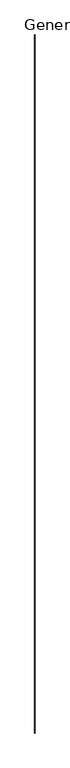
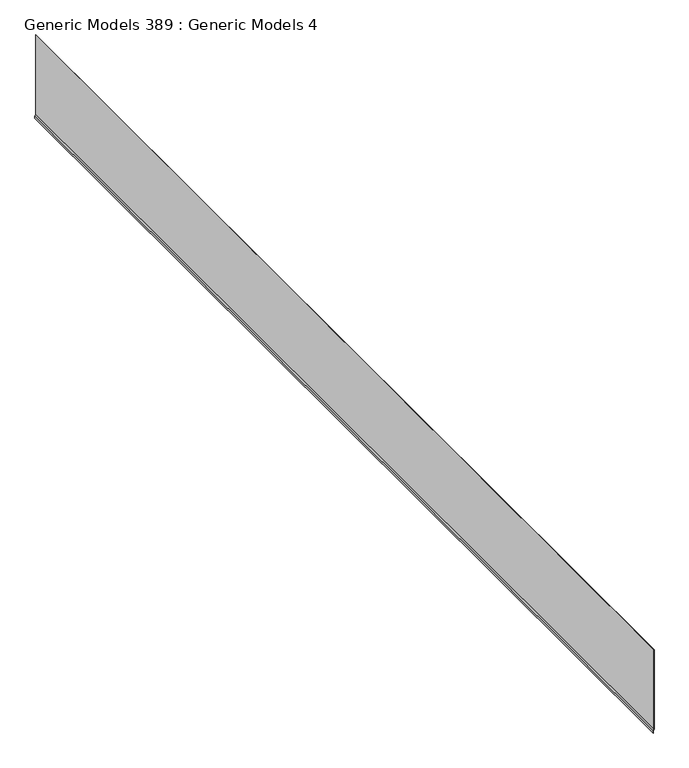
"""IFC4 building model written with IfcOpenShell, lengths in millimetres: proxy geometry, Generic Models 389 : Generic Models 4."""

from ifc_helpers import new_model, si_unit, frame, origin, place, context, project, spatial, polyline, outline, extrude, source, transform, mapped, element, save


def generic_models_389_generic_models_4_7667ba0a(model_context):
    return source(origin(), model_context, "Body", "SweptSolid", [
        extrude(outline(polyline([(126737.3262036, -6624.0173796), (127239.1064906, -6624.0173796), (127239.1064906, -6624.8111296), (126737.4661632, -6624.8111296), (126726.3724169, -6628.848923), (126714.3312142, -6628.848923), (126714.3312142, -6628.055173), (126726.2324574, -6628.055173), (126737.3262036, -6624.0173796)])), frame((0.0, -6864.9230338, 0.0), z_axis=(0.0, 1.0, 0.0), x_axis=(0.0, 0.0, 1.0)), (0.0, 0.0, 1.0), 6400.8),
    ])


if __name__ == "__main__":
    model = new_model("IFC4")
    model_context = context("Model", 3, world=origin())
    ifc_project = project(units=[si_unit("LENGTHUNIT", "METRE", prefix="MILLI")], contexts=[model_context])
    site = spatial("IfcSite", under=ifc_project)
    building = spatial("IfcBuilding", under=site)
    placement = place(None, origin())
    generic_models_389_generic_models_4_shape = generic_models_389_generic_models_4_7667ba0a(model_context)
    element("IfcBuildingElementProxy", 1, Name="Generic Models 389 : Generic Models 4", ObjectType="Generic Models 389 : Generic Models 4", at=placement, inside=building, context=model_context, shape_type="MappedRepresentation", body=[
        mapped(generic_models_389_generic_models_4_shape, transform((0.0, 0.0, 0.0), x_axis=(1.0, 0.0, 0.0), y_axis=(0.0, 1.0, 0.0), z_axis=(0.0, 0.0, 1.0))),
    ])
    save(model, "model.ifc")

# Revit data of these elements
# Element 1 (IfcBuildingElementProxy, "Generic Models 389 : Generic Models 4")
#   Materials on its faces: "_(2) LAYERS NO. 30 ASTM D226 ASPHALT SATURATED ORGANIC FELT"
# Materials
#   "_(2) LAYERS NO. 30 ASTM D226 ASPHALT SATURATED ORGANIC FELT": class "Generic", colour RGB 67 154 161, transparency 0, Cost = 0
